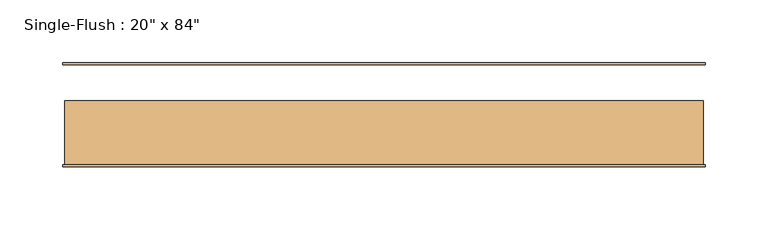
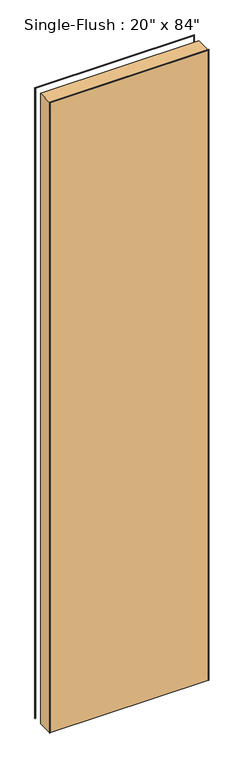
"""IFC4 building model written with IfcOpenShell, lengths in millimetres: door geometry."""

from ifc_helpers import new_model, si_unit, frame, origin, origin_with_axes, place, context, project, spatial, polyline, outline, extrude, source, transform, mapped, element, save


def door_4305e943(model_context):
    return source(origin(), model_context, "Body", "SweptSolid", [
        extrude(outline(polyline([(2135.1875, -255.5875), (0.0, -255.5875), (0.0, -254.0), (2133.6, -254.0), (2133.6, 254.0), (0.0, 254.0), (0.0, 255.5875), (2135.1875, 255.5875), (2135.1875, -255.5875)])), frame((0.0, -41.275, 0.0), z_axis=(0.0, 1.0, 0.0), x_axis=(0.0, 0.0, 1.0)), (0.0, 0.0, 1.0), 1.5875),
        extrude(outline(polyline([(2135.1875, 255.5875), (2135.1875, -255.5875), (0.0, -255.5875), (0.0, -254.0), (2133.6, -254.0), (2133.6, 254.0), (0.0, 254.0), (0.0, 255.5875), (2135.1875, 255.5875)])), frame((0.0, 39.6875, 0.0), z_axis=(0.0, 1.0, 0.0), x_axis=(0.0, 0.0, 1.0)), (0.0, 0.0, 1.0), 1.5875),
        extrude(outline(polyline([(254.0, 11.1125), (254.0, -39.6875), (-254.0, -39.6875), (-254.0, 11.1125), (254.0, 11.1125)])), origin_with_axes(), (0.0, 0.0, 1.0), 2133.6),
    ])


if __name__ == "__main__":
    model = new_model("IFC4")
    model_context = context("Model", 3, world=origin())
    ifc_project = project(units=[si_unit("LENGTHUNIT", "METRE", prefix="MILLI")], contexts=[model_context])
    site = spatial("IfcSite", under=ifc_project)
    building = spatial("IfcBuilding", under=site)
    placement = place(None, origin())
    door_shape = door_4305e943(model_context)
    element("IfcDoor", 1, ObjectType="Single-Flush : 20\" x 84\"", at=placement, inside=building, context=model_context, shape_type="MappedRepresentation", body=[
        mapped(door_shape, transform((0.0, 0.0, 0.0), x_axis=(1.0, 0.0, 0.0), y_axis=(0.0, 1.0, 0.0), z_axis=(0.0, 0.0, 1.0))),
    ])
    save(model, "model.ifc")

# Revit data of these elements
# Type "Single-Flush : 20\" x 84\""
#   Type Mark = "42"
#   Assembly Code = "C1020"
#   Thickness = 0' - 2"
#   Height = 7' - 0"
#   Trim Projection Ext = 0' - 0 1/16"
#   Trim Projection Int = 0' - 0 1/16"
#   Trim Width = 0' - 0 1/16"
#   Width = 1' - 8"
#   Door Material = Door - Panel
#   Frame Material = Door - Frame
#   Function = (empty or 0)
#   Wall Closure = (empty or 0)
# Element 1 (IfcDoor, "Single-Flush : 20\" x 84\"")
#   Materials on its faces: "Door - Frame", "Door - Panel"
# Materials
#   "Door - Panel": class "Wood", colour RGB 210 159 95, transparency 0
#   "Door - Frame": class "Miscellaneous", colour RGB 118 70 51, transparency 0
